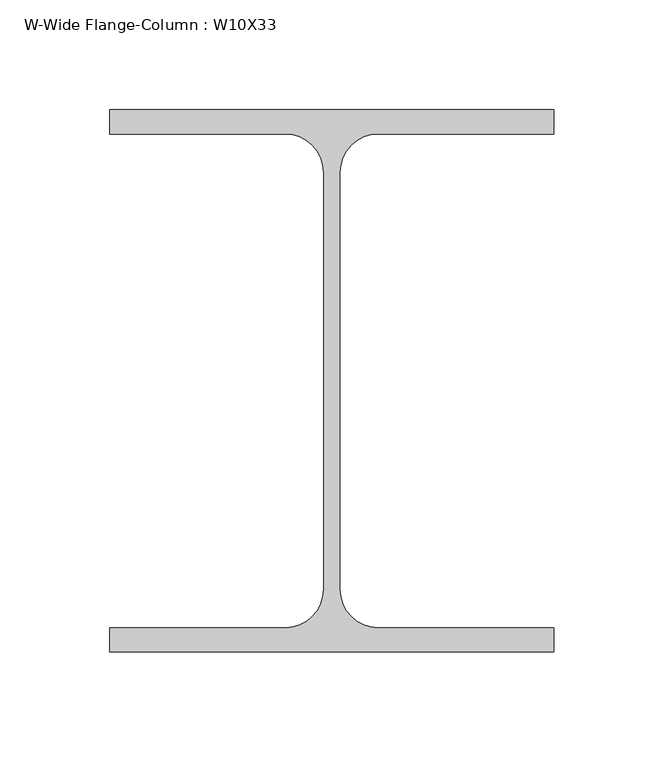
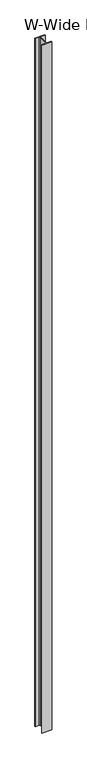
"""IFC4 building model written with IfcOpenShell, lengths in millimetres: column geometry, W-Wide Flange-Column : W10X33."""

from ifc_helpers import new_model, si_unit, point, frame, frame_2d, origin, place, context, project, spatial, polyline, circle_curve, trimmed, segment, composite_curve, outline, extrude, source, transform, mapped, element, save


def w_wide_flange_column_w10x33_e941acc0(model_context):
    return source(origin(), model_context, "Body", "SweptSolid", [
        extrude(outline(composite_curve([segment(polyline([(101.092, 123.571), (101.092, 112.522), (21.209, 112.522)]), True, "CONTINUOUS"), segment(trimmed(circle_curve(frame_2d((21.209, 94.996)), 17.526), [point((21.209, 112.522))], [point((3.683, 94.996))], True, "CARTESIAN"), True, "CONTINUOUS"), segment(polyline([(3.683, 94.996), (3.683, -94.996)]), True, "CONTINUOUS"), segment(trimmed(circle_curve(frame_2d((21.209, -94.996)), 17.526), [point((3.683, -94.996))], [point((21.209, -112.522))], True, "CARTESIAN"), True, "CONTINUOUS"), segment(polyline([(21.209, -112.522), (101.092, -112.522), (101.092, -123.571), (-101.092, -123.571), (-101.092, -112.522), (-21.209, -112.522)]), True, "CONTINUOUS"), segment(trimmed(circle_curve(frame_2d((-21.209, -94.996)), 17.526), [point((-21.209, -112.522))], [point((-3.683, -94.996))], True, "CARTESIAN"), True, "CONTINUOUS"), segment(polyline([(-3.683, -94.996), (-3.683, 94.996)]), True, "CONTINUOUS"), segment(trimmed(circle_curve(frame_2d((-21.209, 94.996)), 17.526), [point((-3.683, 94.996))], [point((-21.209, 112.522))], True, "CARTESIAN"), True, "CONTINUOUS"), segment(polyline([(-21.209, 112.522), (-101.092, 112.522), (-101.092, 123.571), (101.092, 123.571)]), True, "CONTINUOUS")], self_intersect=False)), frame((0.0, 0.0, 12566.65), z_axis=(0.0, 0.0, 1.0), x_axis=(1.0, 0.0, 0.0)), (0.0, 0.0, 1.0), 15017.75),
    ])


if __name__ == "__main__":
    model = new_model("IFC4")
    model_context = context("Model", 3, world=origin())
    ifc_project = project(units=[si_unit("LENGTHUNIT", "METRE", prefix="MILLI")], contexts=[model_context])
    site = spatial("IfcSite", under=ifc_project)
    building = spatial("IfcBuilding", under=site)
    placement = place(None, origin())
    w_wide_flange_column_w10x33_shape = w_wide_flange_column_w10x33_e941acc0(model_context)
    element("IfcColumn", 1, ObjectType="W-Wide Flange-Column : W10X33", at=placement, inside=building, context=model_context, shape_type="MappedRepresentation", body=[
        mapped(w_wide_flange_column_w10x33_shape, transform((0.0, 0.0, 0.0), x_axis=(1.0, 0.0, 0.0), y_axis=(0.0, 1.0, 0.0), z_axis=(0.0, 0.0, 1.0))),
    ])
    save(model, "model.ifc")

# Revit data of these elements
# Type "W-Wide Flange-Column : W10X33"
#   Assembly Code = "B10"
#   W = 33
#   bf = 0' - 7.96"
#   d = 0' - 9.73"
#   k = 0' - 1 1/8"
#   kr = 0' - 0.69"
#   tf = 0' - 0.435"
#   tw = 0' - 0.29"
#   A = 0.0674306 SF
#   Structural Material [instance default] = Steel ASTM A992
# Element 1 (IfcColumn, "W-Wide Flange-Column : W10X33")
#   Materials on its faces: "Steel ASTM A992"
# Materials
#   "Steel ASTM A992": class "Metal", colour RGB 199 199 199, transparency 0, Description = "Structural steel 50ksi", Cost = 0
